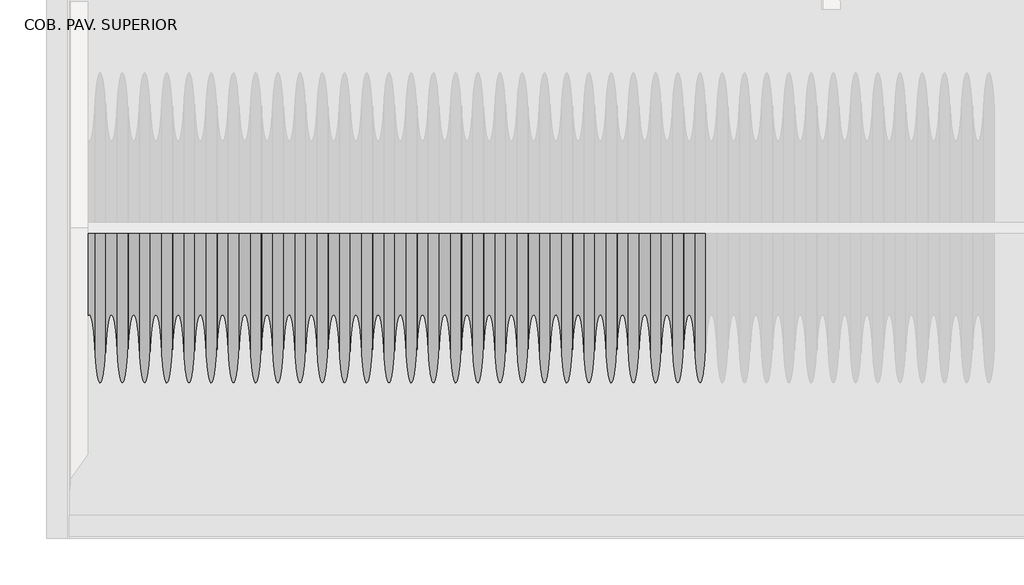
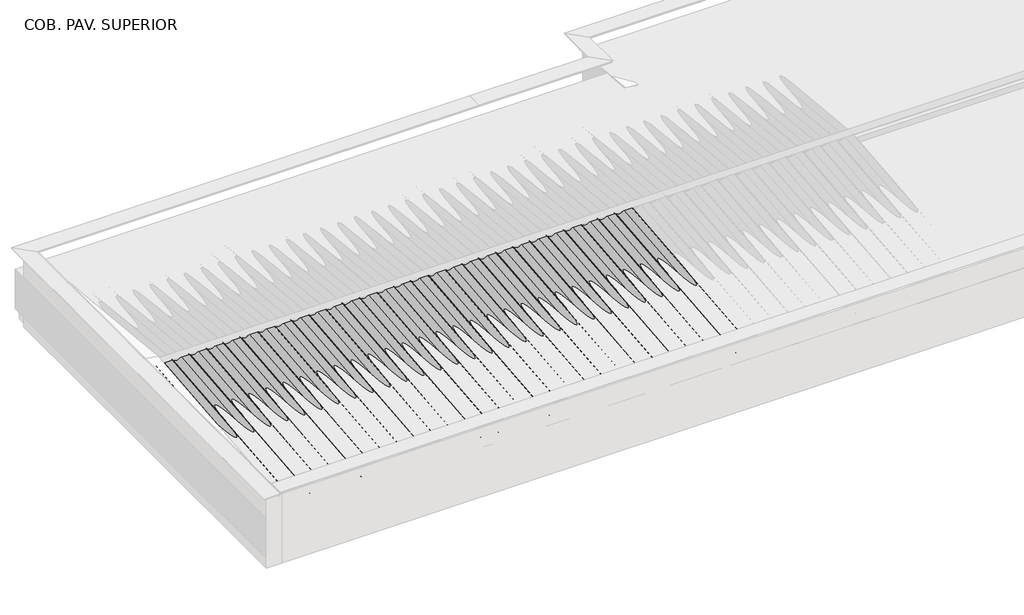
# One storey, part 2 of 8: 35 beams, 7 columns.
"""IFC4 building model written with IfcOpenShell, lengths in millimetres."""

import ifcopenshell
import ifcopenshell.guid

model = None  # the IFC model being written
_history = None  # IfcOwnerHistory: only IFC2X3 demands one
_inside = {}  # id of a spatial element -> (the spatial element, [elements in it])
_under = {}  # id of a project, library or spatial element -> (it, [spatial elements below it])
_declared = {}  # id of a project -> (the project, [libraries it declares])
_typed = {}  # id of a type object -> (the type object, [elements of that type])
_made_of = {}  # id of a material, layer set ... -> (it, [elements and type objects made of it])


def new_model(schema):
    """Start an empty IFC model of exactly this schema.

    Asked for "IFC4X3", IfcOpenShell would pick the latest addendum, in which some entities
    have other attributes; the version numbers below select the first issue.
    IFC2X3 requires an IfcOwnerHistory on every rooted entity: one is made here for all.
    """
    global model, _history
    if schema == "IFC4X3":
        model = ifcopenshell.file(schema_version=(4, 3, 0, 0))
    else:
        model = ifcopenshell.file(schema=schema)
    _inside.clear()
    _under.clear()
    _declared.clear()
    _typed.clear()
    _made_of.clear()
    _history = None
    if model.schema == "IFC2X3":
        org = make("IfcOrganization", Name="unknown")
        user = make(
            "IfcPersonAndOrganization",
            ThePerson=make("IfcPerson", FamilyName="unknown"),
            TheOrganization=org,
        )
        app = make(
            "IfcApplication",
            ApplicationDeveloper=org,
            Version="unknown",
            ApplicationFullName="unknown",
            ApplicationIdentifier="unknown",
        )
        _history = make(
            "IfcOwnerHistory",
            OwningUser=user,
            OwningApplication=app,
            ChangeAction="ADDED",
            CreationDate=0,
        )
    return model


def make(cls, **values):
    """One entity of the class cls with the attributes given. An attribute that is None is left unset."""
    return model.create_entity(
        cls, **{name: value for name, value in values.items() if value is not None}
    )


def rooted(cls, **values):
    """An entity with a GlobalId (a new one), such as an element, a storey or a relation."""
    return make(cls, GlobalId=ifcopenshell.guid.new(), OwnerHistory=_history, **values)


def si_unit(unit_type, name, prefix=None):
    """IfcSIUnit, for example si_unit("LENGTHUNIT", "METRE", prefix="MILLI")."""
    return make("IfcSIUnit", UnitType=unit_type, Prefix=prefix, Name=name)


def assignment(units):
    """IfcUnitAssignment: the units of a project."""
    return None if units is None else make("IfcUnitAssignment", Units=units)


def point(xyz):
    """IfcCartesianPoint."""
    return None if xyz is None else make("IfcCartesianPoint", Coordinates=xyz)


def direction(xyz):
    """IfcDirection."""
    return None if xyz is None else make("IfcDirection", DirectionRatios=xyz)


def frame(location, z_axis=None, x_axis=None):
    """IfcAxis2Placement3D, a coordinate frame: its origin and axes. An axis left out is left unset."""
    return make(
        "IfcAxis2Placement3D",
        Location=point(location),
        Axis=direction(z_axis),
        RefDirection=direction(x_axis),
    )


def frame_2d(location, x_axis=None):
    """IfcAxis2Placement2D, a coordinate frame in the plane: its origin and x axis."""
    return make(
        "IfcAxis2Placement2D", Location=point(location), RefDirection=direction(x_axis)
    )


def origin():
    """The frame at (0, 0, 0) with its axes left unset."""
    return frame((0.0, 0.0, 0.0))


def place(relative_to, where):
    """IfcLocalPlacement: puts the frame where relative to a parent placement (None: the world)."""
    return make(
        "IfcLocalPlacement", PlacementRelTo=relative_to, RelativePlacement=where
    )


def context(
    kind, dimensions, precision=None, world=None, true_north=None, identifier=None
):
    """IfcGeometricRepresentationContext, for example the 3D "Model" context."""
    return make(
        "IfcGeometricRepresentationContext",
        ContextIdentifier=identifier,
        ContextType=kind,
        CoordinateSpaceDimension=dimensions,
        Precision=precision,
        WorldCoordinateSystem=world,
        TrueNorth=true_north,
    )


def project(units=None, contexts=None):
    """IfcProject with its units and contexts."""
    return rooted(
        "IfcProject",
        Name="project",
        RepresentationContexts=contexts,
        UnitsInContext=assignment(units),
    )


def spatial(cls, under=None, at=None, **own):
    """A site, building, storey or space (cls), placed at a placement, below another one or the project."""
    s = rooted(cls, ObjectPlacement=at, **own)
    if under is not None:
        _under.setdefault(under.id(), (under, []))[1].append(s)
    return s


def polyline(points):
    """IfcPolyline through the points."""
    return make("IfcPolyline", Points=[point(p) for p in points])


def circle_curve(where, radius):
    """IfcCircle in the frame where."""
    return make("IfcCircle", Position=where, Radius=radius)


def trimmed(basis, trim1, trim2, sense, master):
    """IfcTrimmedCurve: the piece of a basis curve between two trims."""
    return make(
        "IfcTrimmedCurve",
        BasisCurve=basis,
        Trim1=trim1,
        Trim2=trim2,
        SenseAgreement=sense,
        MasterRepresentation=master,
    )


def segment(curve, same_sense, transition):
    """IfcCompositeCurveSegment."""
    return make(
        "IfcCompositeCurveSegment",
        Transition=transition,
        SameSense=same_sense,
        ParentCurve=curve,
    )


def composite_curve(segments, self_intersect=None):
    """IfcCompositeCurve: segments joined end to end."""
    return make("IfcCompositeCurve", Segments=segments, SelfIntersect=self_intersect)


def outline(outer, holes=None, kind="AREA"):
    """IfcArbitraryClosedProfileDef: a profile drawn as a closed curve; with holes, ...WithVoids."""
    if holes is None:
        return make("IfcArbitraryClosedProfileDef", ProfileType=kind, OuterCurve=outer)
    return make(
        "IfcArbitraryProfileDefWithVoids",
        ProfileType=kind,
        OuterCurve=outer,
        InnerCurves=holes,
    )


def extrude(swept, where, along, depth):
    """IfcExtrudedAreaSolid: the profile swept, set in the frame where, extruded along a direction by depth."""
    return make(
        "IfcExtrudedAreaSolid",
        SweptArea=swept,
        Position=where,
        ExtrudedDirection=direction(along),
        Depth=depth,
    )


def shape(context_of_items, identifier, shape_type, items):
    """IfcShapeRepresentation: the items that make up one representation, for example the "Body"."""
    return make(
        "IfcShapeRepresentation",
        ContextOfItems=context_of_items,
        RepresentationIdentifier=identifier,
        RepresentationType=shape_type,
        Items=items,
    )


def source(mapping_origin, context_of_items, identifier, shape_type, items):
    """IfcRepresentationMap: a shape defined once, which mapped items show again and again."""
    return make(
        "IfcRepresentationMap",
        MappingOrigin=mapping_origin,
        MappedRepresentation=shape(context_of_items, identifier, shape_type, items),
    )


def transform(
    local_origin,
    x_axis=None,
    y_axis=None,
    z_axis=None,
    scale=None,
    scale2=None,
    scale3=None,
    uniform=True,
):
    """IfcCartesianTransformationOperator3D, or its non-uniform kind. x_axis, y_axis, z_axis: its Axis1, 2, 3."""
    if uniform:
        return make(
            "IfcCartesianTransformationOperator3D",
            Axis1=direction(x_axis),
            Axis2=direction(y_axis),
            LocalOrigin=point(local_origin),
            Scale=scale,
            Axis3=direction(z_axis),
        )
    return make(
        "IfcCartesianTransformationOperator3DnonUniform",
        Axis1=direction(x_axis),
        Axis2=direction(y_axis),
        LocalOrigin=point(local_origin),
        Scale=scale,
        Axis3=direction(z_axis),
        Scale2=scale2,
        Scale3=scale3,
    )


def mapped(mapping_source, mapping_target):
    """IfcMappedItem: shows the shape of a source again, moved by a transform."""
    return make(
        "IfcMappedItem", MappingSource=mapping_source, MappingTarget=mapping_target
    )


def made_of(thing, what):
    """Note that an element or type object is made of a material, layer set ...; save() writes the relation."""
    if what is not None:
        _made_of.setdefault(what.id(), (what, []))[1].append(thing)
    return thing


def element(
    cls,
    number,
    at=None,
    inside=None,
    cuts=None,
    type_object=None,
    material=None,
    context=None,
    identifier="Body",
    shape_type=None,
    held_by="IfcProductDefinitionShape",
    body=None,
    shapes=None,
    **own,
):
    """One element of the class cls, such as IfcWall. Its Tag is "e" and its number.

    at: its placement. inside: the storey or other place that contains it. cuts: it is an
    opening in that element (IfcRelVoidsElement). A single representation is given by context,
    identifier, shape_type and body (its items); several are given by shapes. held_by: the class
    of the entity that holds the representations. save() writes the other relations.
    """
    e = rooted(cls, Tag="e%d" % number, ObjectPlacement=at, **own)
    if body is not None:
        shapes = [shape(context, identifier, shape_type, body)]
    if shapes is not None:
        e.Representation = make(held_by, Representations=shapes)
    if inside is not None:
        _inside.setdefault(inside.id(), (inside, []))[1].append(e)
    if cuts is not None:
        rooted(
            "IfcRelVoidsElement", RelatingBuildingElement=cuts, RelatedOpeningElement=e
        )
    if type_object is not None:
        _typed.setdefault(type_object.id(), (type_object, []))[1].append(e)
    return made_of(e, material)


def aggregate(whole, parts):
    """IfcRelAggregates: a whole, such as a stair, and the parts it consists of."""
    return rooted("IfcRelAggregates", RelatingObject=whole, RelatedObjects=parts)


def save(model, path):
    """Write the relations noted so far, then the file.

    IfcRelAggregates (storeys below a building ...), IfcRelContainedInSpatialStructure (elements
    in a storey), IfcRelDefinesByType, IfcRelAssociatesMaterial and IfcRelDeclares: one each for
    every whole, place, type object, material and project.
    """
    for whole, parts in _under.values():
        aggregate(whole, parts)
    for where, things in _inside.values():
        rooted(
            "IfcRelContainedInSpatialStructure",
            RelatedElements=things,
            RelatingStructure=where,
        )
    for kind, things in _typed.values():
        rooted("IfcRelDefinesByType", RelatedObjects=things, RelatingType=kind)
    for what, things in _made_of.values():
        rooted("IfcRelAssociatesMaterial", RelatedObjects=things, RelatingMaterial=what)
    for by, libraries in _declared.values():
        rooted("IfcRelDeclares", RelatingContext=by, RelatedDefinitions=libraries)
    model.write(path)


def beam_fe4ddbad(model_context):
    return source(origin(), model_context, "Body", "SweptSolid", [
        extrude(outline(polyline([(998.8971968, 30.0), (998.8971968, -30.0), (-998.8971974, -30.0), (-998.8971974, 30.0), (998.8971968, 30.0)])), frame((0.0, 0.0, -60.0), z_axis=(0.0, 0.0, 1.0), x_axis=(1.0, 0.0, 0.0)), (0.0, 0.0, 1.0), 120.0),
    ])


def column_6c15bf79(model_context):
    return source(origin(), model_context, "Body", "SweptSolid", [
        extrude(outline(polyline([(30.0, 80.0), (30.0, -80.0), (-30.0, -80.0), (-30.0, 80.0), (30.0, 80.0)])), frame((0.0, 0.0, 6710.0), z_axis=(0.0, 0.0, 1.0), x_axis=(1.0, 0.0, 0.0)), (0.0, 0.0, 1.0), 467.5),
    ])


def column_42eef9f8(model_context):
    return source(origin(), model_context, "Body", "SweptSolid", [
        extrude(outline(polyline([(30.0, 80.0), (30.0, -80.0), (-30.0, -80.0), (-30.0, 80.0), (30.0, 80.0)])), frame((0.0, 0.0, 6710.0), z_axis=(0.0, 0.0, 1.0), x_axis=(1.0, 0.0, 0.0)), (0.0, 0.0, 1.0), 227.1),
    ])


model = new_model("IFC4")

# Units and contexts
model_context = context("Model", 3, world=origin())
ifc_project = project(units=[si_unit("LENGTHUNIT", "METRE", prefix="MILLI")], contexts=[model_context])

# Site, building, storey
site = spatial("IfcSite", under=ifc_project)
building = spatial("IfcBuilding", under=site)
storey = spatial("IfcBuildingStorey", under=building, Name="COB. PAV. SUPERIOR", Elevation=6650.0)

# Beams
placement = place(None, origin())
beam_shape = beam_fe4ddbad(model_context)
element("IfcBeam", 1, ObjectType="Madeira de lei : Berço 6x12cm", at=placement, inside=storey, context=model_context, shape_type="MappedRepresentation", body=[
    mapped(beam_shape, transform((-11738.1841096, -9189.768869, 6680.0), x_axis=(1.0, 0.0, 0.0), y_axis=(0.0, 0.0, -1.0), z_axis=(0.0, 1.0, 0.0))),
])
element("IfcBeam", 2, ObjectType="Madeira de lei : Berço 6x12cm", at=placement, inside=storey, context=model_context, shape_type="MappedRepresentation", body=[
    mapped(beam_shape, transform((-11738.1841096, -10631.818869, 6680.0), x_axis=(1.0, 0.0, 0.0), y_axis=(0.0, 0.0, -1.0), z_axis=(0.0, 1.0, 0.0))),
])
element("IfcBeam", 3, ObjectType="Madeira de lei : Berço 6x12cm", at=placement, inside=storey, context=model_context, shape_type="MappedRepresentation", body=[
    mapped(beam_shape, transform((-9740.3897147, -9189.768869, 6680.0), x_axis=(1.0, 0.0, 0.0), y_axis=(0.0, 0.0, -1.0), z_axis=(0.0, 1.0, 0.0))),
])
element("IfcBeam", 4, ObjectType="Madeira de lei : Berço 6x12cm", at=placement, inside=storey, context=model_context, shape_type="MappedRepresentation", body=[
    mapped(beam_shape, transform((-7742.5953199, -9189.768869, 6680.0), x_axis=(1.0, 0.0, 0.0), y_axis=(0.0, 0.0, -1.0), z_axis=(0.0, 1.0, 0.0))),
])
element("IfcBeam", 5, ObjectType="Madeira de lei : Berço 6x12cm", at=placement, inside=storey, context=model_context, shape_type="MappedRepresentation", body=[
    mapped(beam_shape, transform((-9740.3897147, -10631.818869, 6680.0), x_axis=(1.0, 0.0, 0.0), y_axis=(0.0, 0.0, -1.0), z_axis=(0.0, 1.0, 0.0))),
])
element("IfcBeam", 6, ObjectType="Madeira de lei : Berço 6x12cm", at=placement, inside=storey, context=model_context, shape_type="MappedRepresentation", body=[
    mapped(beam_shape, transform((-7742.5953199, -10631.818869, 6680.0), x_axis=(1.0, 0.0, 0.0), y_axis=(0.0, 0.0, -1.0), z_axis=(0.0, 1.0, 0.0))),
])
element("IfcBeam", 7, ObjectType="Madeira de lei : Berço 6x12cm", at=placement, inside=storey, context=model_context, shape_type="MappedRepresentation", body=[
    mapped(beam_shape, transform((-5744.8009251, -10631.818869, 6680.0), x_axis=(1.0, 0.0, 0.0), y_axis=(0.0, 0.0, -1.0), z_axis=(0.0, 1.0, 0.0))),
])
element("IfcBeam", 8, ObjectType="Telha Ondulada : Fibrocimento", at=placement, inside=storey, context=model_context, shape_type="SweptSolid", body=[
    extrude(outline(composite_curve([segment(trimmed(circle_curve(frame_2d((0.0, 66.7939461)), 66.7939461), [point((29.3501489, 6.7939461))], [point((29.3501489, 126.7939461))], True, "CARTESIAN"), True, "CONTINUOUS"), segment(polyline([(29.3501489, 126.7939461), (31.5472154, 131.2853711)]), True, "CONTINUOUS"), segment(trimmed(circle_curve(frame_2d((0.0, 66.7939461)), 71.7939461), [point((31.5472154, 131.2853711))], [point((31.5472154, 2.3025211))], False, "CARTESIAN"), True, "CONTINUOUS"), segment(trimmed(circle_curve(frame_2d((58.7002978, -53.2060539)), 61.7939461), [point((31.5472154, 2.3025211))], [point((31.5472154, -108.7146289))], True, "CARTESIAN"), True, "CONTINUOUS"), segment(polyline([(31.5472154, -108.7146289), (29.3501489, -113.2060539)]), True, "CONTINUOUS"), segment(trimmed(circle_curve(frame_2d((58.7002978, -53.2060539)), 66.7939461), [point((29.3501489, -113.2060539))], [point((29.3501489, 6.7939461))], False, "CARTESIAN"), True, "CONTINUOUS")], self_intersect=False)), frame((-12452.7843743, -10831.9594023, 7106.8215886), z_axis=(0.0, 0.9950371902099894, 0.09950371902099749), x_axis=(0.0, 0.09950371902099749, -0.9950371902099894)), (0.0, 0.0, 1.0), 3060.4439799),
])
element("IfcBeam", 9, ObjectType="Telha Ondulada : Fibrocimento", at=placement, inside=storey, context=model_context, shape_type="SweptSolid", body=[
    extrude(outline(composite_curve([segment(trimmed(circle_curve(frame_2d((0.0, 66.7939461)), 66.7939461), [point((29.3501489, 6.7939461))], [point((29.3501489, 126.7939461))], True, "CARTESIAN"), True, "CONTINUOUS"), segment(polyline([(29.3501489, 126.7939461), (31.5472154, 131.2853711)]), True, "CONTINUOUS"), segment(trimmed(circle_curve(frame_2d((0.0, 66.7939461)), 71.7939461), [point((31.5472154, 131.2853711))], [point((31.5472154, 2.3025211))], False, "CARTESIAN"), True, "CONTINUOUS"), segment(trimmed(circle_curve(frame_2d((58.7002978, -53.2060539)), 61.7939461), [point((31.5472154, 2.3025211))], [point((31.5472154, -108.7146289))], True, "CARTESIAN"), True, "CONTINUOUS"), segment(polyline([(31.5472154, -108.7146289), (29.3501489, -113.2060539)]), True, "CONTINUOUS"), segment(trimmed(circle_curve(frame_2d((58.7002978, -53.2060539)), 66.7939461), [point((29.3501489, -113.2060539))], [point((29.3501489, 6.7939461))], False, "CARTESIAN"), True, "CONTINUOUS")], self_intersect=False)), frame((-12208.2843743, -10831.9594023, 7106.8215886), z_axis=(0.0, 0.9950371902099894, 0.09950371902099749), x_axis=(0.0, 0.09950371902099749, -0.9950371902099894)), (0.0, 0.0, 1.0), 3060.4439799),
])
element("IfcBeam", 10, ObjectType="Telha Ondulada : Fibrocimento", at=placement, inside=storey, context=model_context, shape_type="SweptSolid", body=[
    extrude(outline(composite_curve([segment(trimmed(circle_curve(frame_2d((0.0, 66.7939461)), 66.7939461), [point((29.3501489, 6.7939461))], [point((29.3501489, 126.7939461))], True, "CARTESIAN"), True, "CONTINUOUS"), segment(polyline([(29.3501489, 126.7939461), (31.5472154, 131.2853711)]), True, "CONTINUOUS"), segment(trimmed(circle_curve(frame_2d((0.0, 66.7939461)), 71.7939461), [point((31.5472154, 131.2853711))], [point((31.5472154, 2.3025211))], False, "CARTESIAN"), True, "CONTINUOUS"), segment(trimmed(circle_curve(frame_2d((58.7002978, -53.2060539)), 61.7939461), [point((31.5472154, 2.3025211))], [point((31.5472154, -108.7146289))], True, "CARTESIAN"), True, "CONTINUOUS"), segment(polyline([(31.5472154, -108.7146289), (29.3501489, -113.2060539)]), True, "CONTINUOUS"), segment(trimmed(circle_curve(frame_2d((58.7002978, -53.2060539)), 66.7939461), [point((29.3501489, -113.2060539))], [point((29.3501489, 6.7939461))], False, "CARTESIAN"), True, "CONTINUOUS")], self_intersect=False)), frame((-11963.7843743, -10831.9594023, 7106.8215886), z_axis=(0.0, 0.9950371902099894, 0.09950371902099749), x_axis=(0.0, 0.09950371902099749, -0.9950371902099894)), (0.0, 0.0, 1.0), 3060.4439799),
])
element("IfcBeam", 11, ObjectType="Telha Ondulada : Fibrocimento", at=placement, inside=storey, context=model_context, shape_type="SweptSolid", body=[
    extrude(outline(composite_curve([segment(trimmed(circle_curve(frame_2d((0.0, 66.7939461)), 66.7939461), [point((29.3501489, 6.7939461))], [point((29.3501489, 126.7939461))], True, "CARTESIAN"), True, "CONTINUOUS"), segment(polyline([(29.3501489, 126.7939461), (31.5472154, 131.2853711)]), True, "CONTINUOUS"), segment(trimmed(circle_curve(frame_2d((0.0, 66.7939461)), 71.7939461), [point((31.5472154, 131.2853711))], [point((31.5472154, 2.3025211))], False, "CARTESIAN"), True, "CONTINUOUS"), segment(trimmed(circle_curve(frame_2d((58.7002978, -53.2060539)), 61.7939461), [point((31.5472154, 2.3025211))], [point((31.5472154, -108.7146289))], True, "CARTESIAN"), True, "CONTINUOUS"), segment(polyline([(31.5472154, -108.7146289), (29.3501489, -113.2060539)]), True, "CONTINUOUS"), segment(trimmed(circle_curve(frame_2d((58.7002978, -53.2060539)), 66.7939461), [point((29.3501489, -113.2060539))], [point((29.3501489, 6.7939461))], False, "CARTESIAN"), True, "CONTINUOUS")], self_intersect=False)), frame((-11719.2843743, -10831.9594023, 7106.8215886), z_axis=(0.0, 0.9950371902099894, 0.09950371902099749), x_axis=(0.0, 0.09950371902099749, -0.9950371902099894)), (0.0, 0.0, 1.0), 3060.4439799),
])
element("IfcBeam", 12, ObjectType="Telha Ondulada : Fibrocimento", at=placement, inside=storey, context=model_context, shape_type="SweptSolid", body=[
    extrude(outline(composite_curve([segment(trimmed(circle_curve(frame_2d((0.0, 66.7939461)), 66.7939461), [point((29.3501489, 6.7939461))], [point((29.3501489, 126.7939461))], True, "CARTESIAN"), True, "CONTINUOUS"), segment(polyline([(29.3501489, 126.7939461), (31.5472154, 131.2853711)]), True, "CONTINUOUS"), segment(trimmed(circle_curve(frame_2d((0.0, 66.7939461)), 71.7939461), [point((31.5472154, 131.2853711))], [point((31.5472154, 2.3025211))], False, "CARTESIAN"), True, "CONTINUOUS"), segment(trimmed(circle_curve(frame_2d((58.7002978, -53.2060539)), 61.7939461), [point((31.5472154, 2.3025211))], [point((31.5472154, -108.7146289))], True, "CARTESIAN"), True, "CONTINUOUS"), segment(polyline([(31.5472154, -108.7146289), (29.3501489, -113.2060539)]), True, "CONTINUOUS"), segment(trimmed(circle_curve(frame_2d((58.7002978, -53.2060539)), 66.7939461), [point((29.3501489, -113.2060539))], [point((29.3501489, 6.7939461))], False, "CARTESIAN"), True, "CONTINUOUS")], self_intersect=False)), frame((-11474.7843743, -10831.9594023, 7106.8215886), z_axis=(0.0, 0.9950371902099894, 0.09950371902099749), x_axis=(0.0, 0.09950371902099749, -0.9950371902099894)), (0.0, 0.0, 1.0), 3060.4439799),
])
element("IfcBeam", 13, ObjectType="Telha Ondulada : Fibrocimento", at=placement, inside=storey, context=model_context, shape_type="SweptSolid", body=[
    extrude(outline(composite_curve([segment(trimmed(circle_curve(frame_2d((0.0, 66.7939461)), 66.7939461), [point((29.3501489, 6.7939461))], [point((29.3501489, 126.7939461))], True, "CARTESIAN"), True, "CONTINUOUS"), segment(polyline([(29.3501489, 126.7939461), (31.5472154, 131.2853711)]), True, "CONTINUOUS"), segment(trimmed(circle_curve(frame_2d((0.0, 66.7939461)), 71.7939461), [point((31.5472154, 131.2853711))], [point((31.5472154, 2.3025211))], False, "CARTESIAN"), True, "CONTINUOUS"), segment(trimmed(circle_curve(frame_2d((58.7002978, -53.2060539)), 61.7939461), [point((31.5472154, 2.3025211))], [point((31.5472154, -108.7146289))], True, "CARTESIAN"), True, "CONTINUOUS"), segment(polyline([(31.5472154, -108.7146289), (29.3501489, -113.2060539)]), True, "CONTINUOUS"), segment(trimmed(circle_curve(frame_2d((58.7002978, -53.2060539)), 66.7939461), [point((29.3501489, -113.2060539))], [point((29.3501489, 6.7939461))], False, "CARTESIAN"), True, "CONTINUOUS")], self_intersect=False)), frame((-11230.2843743, -10831.9594023, 7106.8215886), z_axis=(0.0, 0.9950371902099894, 0.09950371902099749), x_axis=(0.0, 0.09950371902099749, -0.9950371902099894)), (0.0, 0.0, 1.0), 3060.4439799),
])
element("IfcBeam", 14, ObjectType="Telha Ondulada : Fibrocimento", at=placement, inside=storey, context=model_context, shape_type="SweptSolid", body=[
    extrude(outline(composite_curve([segment(trimmed(circle_curve(frame_2d((0.0, 66.7939461)), 66.7939461), [point((29.3501489, 6.7939461))], [point((29.3501489, 126.7939461))], True, "CARTESIAN"), True, "CONTINUOUS"), segment(polyline([(29.3501489, 126.7939461), (31.5472154, 131.2853711)]), True, "CONTINUOUS"), segment(trimmed(circle_curve(frame_2d((0.0, 66.7939461)), 71.7939461), [point((31.5472154, 131.2853711))], [point((31.5472154, 2.3025211))], False, "CARTESIAN"), True, "CONTINUOUS"), segment(trimmed(circle_curve(frame_2d((58.7002978, -53.2060539)), 61.7939461), [point((31.5472154, 2.3025211))], [point((31.5472154, -108.7146289))], True, "CARTESIAN"), True, "CONTINUOUS"), segment(polyline([(31.5472154, -108.7146289), (29.3501489, -113.2060539)]), True, "CONTINUOUS"), segment(trimmed(circle_curve(frame_2d((58.7002978, -53.2060539)), 66.7939461), [point((29.3501489, -113.2060539))], [point((29.3501489, 6.7939461))], False, "CARTESIAN"), True, "CONTINUOUS")], self_intersect=False)), frame((-10985.7843743, -10831.9594023, 7106.8215886), z_axis=(0.0, 0.9950371902099894, 0.09950371902099749), x_axis=(0.0, 0.09950371902099749, -0.9950371902099894)), (0.0, 0.0, 1.0), 3060.4439799),
])
element("IfcBeam", 15, ObjectType="Telha Ondulada : Fibrocimento", at=placement, inside=storey, context=model_context, shape_type="SweptSolid", body=[
    extrude(outline(composite_curve([segment(trimmed(circle_curve(frame_2d((0.0, 66.7939461)), 66.7939461), [point((29.3501489, 6.7939461))], [point((29.3501489, 126.7939461))], True, "CARTESIAN"), True, "CONTINUOUS"), segment(polyline([(29.3501489, 126.7939461), (31.5472154, 131.2853711)]), True, "CONTINUOUS"), segment(trimmed(circle_curve(frame_2d((0.0, 66.7939461)), 71.7939461), [point((31.5472154, 131.2853711))], [point((31.5472154, 2.3025211))], False, "CARTESIAN"), True, "CONTINUOUS"), segment(trimmed(circle_curve(frame_2d((58.7002978, -53.2060539)), 61.7939461), [point((31.5472154, 2.3025211))], [point((31.5472154, -108.7146289))], True, "CARTESIAN"), True, "CONTINUOUS"), segment(polyline([(31.5472154, -108.7146289), (29.3501489, -113.2060539)]), True, "CONTINUOUS"), segment(trimmed(circle_curve(frame_2d((58.7002978, -53.2060539)), 66.7939461), [point((29.3501489, -113.2060539))], [point((29.3501489, 6.7939461))], False, "CARTESIAN"), True, "CONTINUOUS")], self_intersect=False)), frame((-10741.2843743, -10831.9594023, 7106.8215886), z_axis=(0.0, 0.9950371902099894, 0.09950371902099749), x_axis=(0.0, 0.09950371902099749, -0.9950371902099894)), (0.0, 0.0, 1.0), 3060.4439799),
])
element("IfcBeam", 16, ObjectType="Telha Ondulada : Fibrocimento", at=placement, inside=storey, context=model_context, shape_type="SweptSolid", body=[
    extrude(outline(composite_curve([segment(trimmed(circle_curve(frame_2d((0.0, 66.7939461)), 66.7939461), [point((29.3501489, 6.7939461))], [point((29.3501489, 126.7939461))], True, "CARTESIAN"), True, "CONTINUOUS"), segment(polyline([(29.3501489, 126.7939461), (31.5472154, 131.2853711)]), True, "CONTINUOUS"), segment(trimmed(circle_curve(frame_2d((0.0, 66.7939461)), 71.7939461), [point((31.5472154, 131.2853711))], [point((31.5472154, 2.3025211))], False, "CARTESIAN"), True, "CONTINUOUS"), segment(trimmed(circle_curve(frame_2d((58.7002978, -53.2060539)), 61.7939461), [point((31.5472154, 2.3025211))], [point((31.5472154, -108.7146289))], True, "CARTESIAN"), True, "CONTINUOUS"), segment(polyline([(31.5472154, -108.7146289), (29.3501489, -113.2060539)]), True, "CONTINUOUS"), segment(trimmed(circle_curve(frame_2d((58.7002978, -53.2060539)), 66.7939461), [point((29.3501489, -113.2060539))], [point((29.3501489, 6.7939461))], False, "CARTESIAN"), True, "CONTINUOUS")], self_intersect=False)), frame((-10496.7843743, -10831.9594023, 7106.8215886), z_axis=(0.0, 0.9950371902099894, 0.09950371902099749), x_axis=(0.0, 0.09950371902099749, -0.9950371902099894)), (0.0, 0.0, 1.0), 3060.4439799),
])
element("IfcBeam", 17, ObjectType="Telha Ondulada : Fibrocimento", at=placement, inside=storey, context=model_context, shape_type="SweptSolid", body=[
    extrude(outline(composite_curve([segment(trimmed(circle_curve(frame_2d((0.0, 66.7939461)), 66.7939461), [point((29.3501489, 6.7939461))], [point((29.3501489, 126.7939461))], True, "CARTESIAN"), True, "CONTINUOUS"), segment(polyline([(29.3501489, 126.7939461), (31.5472154, 131.2853711)]), True, "CONTINUOUS"), segment(trimmed(circle_curve(frame_2d((0.0, 66.7939461)), 71.7939461), [point((31.5472154, 131.2853711))], [point((31.5472154, 2.3025211))], False, "CARTESIAN"), True, "CONTINUOUS"), segment(trimmed(circle_curve(frame_2d((58.7002978, -53.2060539)), 61.7939461), [point((31.5472154, 2.3025211))], [point((31.5472154, -108.7146289))], True, "CARTESIAN"), True, "CONTINUOUS"), segment(polyline([(31.5472154, -108.7146289), (29.3501489, -113.2060539)]), True, "CONTINUOUS"), segment(trimmed(circle_curve(frame_2d((58.7002978, -53.2060539)), 66.7939461), [point((29.3501489, -113.2060539))], [point((29.3501489, 6.7939461))], False, "CARTESIAN"), True, "CONTINUOUS")], self_intersect=False)), frame((-10252.2843743, -10831.9594023, 7106.8215886), z_axis=(0.0, 0.9950371902099894, 0.09950371902099749), x_axis=(0.0, 0.09950371902099749, -0.9950371902099894)), (0.0, 0.0, 1.0), 3060.4439799),
])
element("IfcBeam", 18, ObjectType="Telha Ondulada : Fibrocimento", at=placement, inside=storey, context=model_context, shape_type="SweptSolid", body=[
    extrude(outline(composite_curve([segment(trimmed(circle_curve(frame_2d((0.0, 66.7939461)), 66.7939461), [point((29.3501489, 6.7939461))], [point((29.3501489, 126.7939461))], True, "CARTESIAN"), True, "CONTINUOUS"), segment(polyline([(29.3501489, 126.7939461), (31.5472154, 131.2853711)]), True, "CONTINUOUS"), segment(trimmed(circle_curve(frame_2d((0.0, 66.7939461)), 71.7939461), [point((31.5472154, 131.2853711))], [point((31.5472154, 2.3025211))], False, "CARTESIAN"), True, "CONTINUOUS"), segment(trimmed(circle_curve(frame_2d((58.7002978, -53.2060539)), 61.7939461), [point((31.5472154, 2.3025211))], [point((31.5472154, -108.7146289))], True, "CARTESIAN"), True, "CONTINUOUS"), segment(polyline([(31.5472154, -108.7146289), (29.3501489, -113.2060539)]), True, "CONTINUOUS"), segment(trimmed(circle_curve(frame_2d((58.7002978, -53.2060539)), 66.7939461), [point((29.3501489, -113.2060539))], [point((29.3501489, 6.7939461))], False, "CARTESIAN"), True, "CONTINUOUS")], self_intersect=False)), frame((-10007.7843743, -10831.9594023, 7106.8215886), z_axis=(0.0, 0.9950371902099894, 0.09950371902099749), x_axis=(0.0, 0.09950371902099749, -0.9950371902099894)), (0.0, 0.0, 1.0), 3060.4439799),
])
element("IfcBeam", 19, ObjectType="Telha Ondulada : Fibrocimento", at=placement, inside=storey, context=model_context, shape_type="SweptSolid", body=[
    extrude(outline(composite_curve([segment(trimmed(circle_curve(frame_2d((0.0, 66.7939461)), 66.7939461), [point((29.3501489, 6.7939461))], [point((29.3501489, 126.7939461))], True, "CARTESIAN"), True, "CONTINUOUS"), segment(polyline([(29.3501489, 126.7939461), (31.5472154, 131.2853711)]), True, "CONTINUOUS"), segment(trimmed(circle_curve(frame_2d((0.0, 66.7939461)), 71.7939461), [point((31.5472154, 131.2853711))], [point((31.5472154, 2.3025211))], False, "CARTESIAN"), True, "CONTINUOUS"), segment(trimmed(circle_curve(frame_2d((58.7002978, -53.2060539)), 61.7939461), [point((31.5472154, 2.3025211))], [point((31.5472154, -108.7146289))], True, "CARTESIAN"), True, "CONTINUOUS"), segment(polyline([(31.5472154, -108.7146289), (29.3501489, -113.2060539)]), True, "CONTINUOUS"), segment(trimmed(circle_curve(frame_2d((58.7002978, -53.2060539)), 66.7939461), [point((29.3501489, -113.2060539))], [point((29.3501489, 6.7939461))], False, "CARTESIAN"), True, "CONTINUOUS")], self_intersect=False)), frame((-9763.2843743, -10831.9594023, 7106.8215886), z_axis=(0.0, 0.9950371902099894, 0.09950371902099749), x_axis=(0.0, 0.09950371902099749, -0.9950371902099894)), (0.0, 0.0, 1.0), 3060.4439799),
])
element("IfcBeam", 20, ObjectType="Telha Ondulada : Fibrocimento", at=placement, inside=storey, context=model_context, shape_type="SweptSolid", body=[
    extrude(outline(composite_curve([segment(trimmed(circle_curve(frame_2d((0.0, 66.7939461)), 66.7939461), [point((29.3501489, 6.7939461))], [point((29.3501489, 126.7939461))], True, "CARTESIAN"), True, "CONTINUOUS"), segment(polyline([(29.3501489, 126.7939461), (31.5472154, 131.2853711)]), True, "CONTINUOUS"), segment(trimmed(circle_curve(frame_2d((0.0, 66.7939461)), 71.7939461), [point((31.5472154, 131.2853711))], [point((31.5472154, 2.3025211))], False, "CARTESIAN"), True, "CONTINUOUS"), segment(trimmed(circle_curve(frame_2d((58.7002978, -53.2060539)), 61.7939461), [point((31.5472154, 2.3025211))], [point((31.5472154, -108.7146289))], True, "CARTESIAN"), True, "CONTINUOUS"), segment(polyline([(31.5472154, -108.7146289), (29.3501489, -113.2060539)]), True, "CONTINUOUS"), segment(trimmed(circle_curve(frame_2d((58.7002978, -53.2060539)), 66.7939461), [point((29.3501489, -113.2060539))], [point((29.3501489, 6.7939461))], False, "CARTESIAN"), True, "CONTINUOUS")], self_intersect=False)), frame((-9518.7843743, -10831.9594023, 7106.8215886), z_axis=(0.0, 0.9950371902099894, 0.09950371902099749), x_axis=(0.0, 0.09950371902099749, -0.9950371902099894)), (0.0, 0.0, 1.0), 3060.4439799),
])
element("IfcBeam", 21, ObjectType="Telha Ondulada : Fibrocimento", at=placement, inside=storey, context=model_context, shape_type="SweptSolid", body=[
    extrude(outline(composite_curve([segment(trimmed(circle_curve(frame_2d((0.0, 66.7939461)), 66.7939461), [point((29.3501489, 6.7939461))], [point((29.3501489, 126.7939461))], True, "CARTESIAN"), True, "CONTINUOUS"), segment(polyline([(29.3501489, 126.7939461), (31.5472154, 131.2853711)]), True, "CONTINUOUS"), segment(trimmed(circle_curve(frame_2d((0.0, 66.7939461)), 71.7939461), [point((31.5472154, 131.2853711))], [point((31.5472154, 2.3025211))], False, "CARTESIAN"), True, "CONTINUOUS"), segment(trimmed(circle_curve(frame_2d((58.7002978, -53.2060539)), 61.7939461), [point((31.5472154, 2.3025211))], [point((31.5472154, -108.7146289))], True, "CARTESIAN"), True, "CONTINUOUS"), segment(polyline([(31.5472154, -108.7146289), (29.3501489, -113.2060539)]), True, "CONTINUOUS"), segment(trimmed(circle_curve(frame_2d((58.7002978, -53.2060539)), 66.7939461), [point((29.3501489, -113.2060539))], [point((29.3501489, 6.7939461))], False, "CARTESIAN"), True, "CONTINUOUS")], self_intersect=False)), frame((-9274.2843743, -10831.9594023, 7106.8215886), z_axis=(0.0, 0.9950371902099894, 0.09950371902099749), x_axis=(0.0, 0.09950371902099749, -0.9950371902099894)), (0.0, 0.0, 1.0), 3060.4439799),
])
element("IfcBeam", 22, ObjectType="Telha Ondulada : Fibrocimento", at=placement, inside=storey, context=model_context, shape_type="SweptSolid", body=[
    extrude(outline(composite_curve([segment(trimmed(circle_curve(frame_2d((0.0, 66.7939461)), 66.7939461), [point((29.3501489, 6.7939461))], [point((29.3501489, 126.7939461))], True, "CARTESIAN"), True, "CONTINUOUS"), segment(polyline([(29.3501489, 126.7939461), (31.5472154, 131.2853711)]), True, "CONTINUOUS"), segment(trimmed(circle_curve(frame_2d((0.0, 66.7939461)), 71.7939461), [point((31.5472154, 131.2853711))], [point((31.5472154, 2.3025211))], False, "CARTESIAN"), True, "CONTINUOUS"), segment(trimmed(circle_curve(frame_2d((58.7002978, -53.2060539)), 61.7939461), [point((31.5472154, 2.3025211))], [point((31.5472154, -108.7146289))], True, "CARTESIAN"), True, "CONTINUOUS"), segment(polyline([(31.5472154, -108.7146289), (29.3501489, -113.2060539)]), True, "CONTINUOUS"), segment(trimmed(circle_curve(frame_2d((58.7002978, -53.2060539)), 66.7939461), [point((29.3501489, -113.2060539))], [point((29.3501489, 6.7939461))], False, "CARTESIAN"), True, "CONTINUOUS")], self_intersect=False)), frame((-9029.7843743, -10831.9594023, 7106.8215886), z_axis=(0.0, 0.9950371902099894, 0.09950371902099749), x_axis=(0.0, 0.09950371902099749, -0.9950371902099894)), (0.0, 0.0, 1.0), 3060.4439799),
])
element("IfcBeam", 23, ObjectType="Telha Ondulada : Fibrocimento", at=placement, inside=storey, context=model_context, shape_type="SweptSolid", body=[
    extrude(outline(composite_curve([segment(trimmed(circle_curve(frame_2d((0.0, 66.7939461)), 66.7939461), [point((29.3501489, 6.7939461))], [point((29.3501489, 126.7939461))], True, "CARTESIAN"), True, "CONTINUOUS"), segment(polyline([(29.3501489, 126.7939461), (31.5472154, 131.2853711)]), True, "CONTINUOUS"), segment(trimmed(circle_curve(frame_2d((0.0, 66.7939461)), 71.7939461), [point((31.5472154, 131.2853711))], [point((31.5472154, 2.3025211))], False, "CARTESIAN"), True, "CONTINUOUS"), segment(trimmed(circle_curve(frame_2d((58.7002978, -53.2060539)), 61.7939461), [point((31.5472154, 2.3025211))], [point((31.5472154, -108.7146289))], True, "CARTESIAN"), True, "CONTINUOUS"), segment(polyline([(31.5472154, -108.7146289), (29.3501489, -113.2060539)]), True, "CONTINUOUS"), segment(trimmed(circle_curve(frame_2d((58.7002978, -53.2060539)), 66.7939461), [point((29.3501489, -113.2060539))], [point((29.3501489, 6.7939461))], False, "CARTESIAN"), True, "CONTINUOUS")], self_intersect=False)), frame((-8785.2843743, -10831.9594023, 7106.8215886), z_axis=(0.0, 0.9950371902099894, 0.09950371902099749), x_axis=(0.0, 0.09950371902099749, -0.9950371902099894)), (0.0, 0.0, 1.0), 3060.4439799),
])
element("IfcBeam", 24, ObjectType="Telha Ondulada : Fibrocimento", at=placement, inside=storey, context=model_context, shape_type="SweptSolid", body=[
    extrude(outline(composite_curve([segment(trimmed(circle_curve(frame_2d((0.0, 66.7939461)), 66.7939461), [point((29.3501489, 6.7939461))], [point((29.3501489, 126.7939461))], True, "CARTESIAN"), True, "CONTINUOUS"), segment(polyline([(29.3501489, 126.7939461), (31.5472154, 131.2853711)]), True, "CONTINUOUS"), segment(trimmed(circle_curve(frame_2d((0.0, 66.7939461)), 71.7939461), [point((31.5472154, 131.2853711))], [point((31.5472154, 2.3025211))], False, "CARTESIAN"), True, "CONTINUOUS"), segment(trimmed(circle_curve(frame_2d((58.7002978, -53.2060539)), 61.7939461), [point((31.5472154, 2.3025211))], [point((31.5472154, -108.7146289))], True, "CARTESIAN"), True, "CONTINUOUS"), segment(polyline([(31.5472154, -108.7146289), (29.3501489, -113.2060539)]), True, "CONTINUOUS"), segment(trimmed(circle_curve(frame_2d((58.7002978, -53.2060539)), 66.7939461), [point((29.3501489, -113.2060539))], [point((29.3501489, 6.7939461))], False, "CARTESIAN"), True, "CONTINUOUS")], self_intersect=False)), frame((-8540.7843743, -10831.9594023, 7106.8215886), z_axis=(0.0, 0.9950371902099894, 0.09950371902099749), x_axis=(0.0, 0.09950371902099749, -0.9950371902099894)), (0.0, 0.0, 1.0), 3060.4439799),
])
element("IfcBeam", 25, ObjectType="Telha Ondulada : Fibrocimento", at=placement, inside=storey, context=model_context, shape_type="SweptSolid", body=[
    extrude(outline(composite_curve([segment(trimmed(circle_curve(frame_2d((0.0, 66.7939461)), 66.7939461), [point((29.3501489, 6.7939461))], [point((29.3501489, 126.7939461))], True, "CARTESIAN"), True, "CONTINUOUS"), segment(polyline([(29.3501489, 126.7939461), (31.5472154, 131.2853711)]), True, "CONTINUOUS"), segment(trimmed(circle_curve(frame_2d((0.0, 66.7939461)), 71.7939461), [point((31.5472154, 131.2853711))], [point((31.5472154, 2.3025211))], False, "CARTESIAN"), True, "CONTINUOUS"), segment(trimmed(circle_curve(frame_2d((58.7002978, -53.2060539)), 61.7939461), [point((31.5472154, 2.3025211))], [point((31.5472154, -108.7146289))], True, "CARTESIAN"), True, "CONTINUOUS"), segment(polyline([(31.5472154, -108.7146289), (29.3501489, -113.2060539)]), True, "CONTINUOUS"), segment(trimmed(circle_curve(frame_2d((58.7002978, -53.2060539)), 66.7939461), [point((29.3501489, -113.2060539))], [point((29.3501489, 6.7939461))], False, "CARTESIAN"), True, "CONTINUOUS")], self_intersect=False)), frame((-8296.2843743, -10831.9594023, 7106.8215886), z_axis=(0.0, 0.9950371902099894, 0.09950371902099749), x_axis=(0.0, 0.09950371902099749, -0.9950371902099894)), (0.0, 0.0, 1.0), 3060.4439799),
])
element("IfcBeam", 26, ObjectType="Telha Ondulada : Fibrocimento", at=placement, inside=storey, context=model_context, shape_type="SweptSolid", body=[
    extrude(outline(composite_curve([segment(trimmed(circle_curve(frame_2d((0.0, 66.7939461)), 66.7939461), [point((29.3501489, 6.7939461))], [point((29.3501489, 126.7939461))], True, "CARTESIAN"), True, "CONTINUOUS"), segment(polyline([(29.3501489, 126.7939461), (31.5472154, 131.2853711)]), True, "CONTINUOUS"), segment(trimmed(circle_curve(frame_2d((0.0, 66.7939461)), 71.7939461), [point((31.5472154, 131.2853711))], [point((31.5472154, 2.3025211))], False, "CARTESIAN"), True, "CONTINUOUS"), segment(trimmed(circle_curve(frame_2d((58.7002978, -53.2060539)), 61.7939461), [point((31.5472154, 2.3025211))], [point((31.5472154, -108.7146289))], True, "CARTESIAN"), True, "CONTINUOUS"), segment(polyline([(31.5472154, -108.7146289), (29.3501489, -113.2060539)]), True, "CONTINUOUS"), segment(trimmed(circle_curve(frame_2d((58.7002978, -53.2060539)), 66.7939461), [point((29.3501489, -113.2060539))], [point((29.3501489, 6.7939461))], False, "CARTESIAN"), True, "CONTINUOUS")], self_intersect=False)), frame((-8051.7843743, -10831.9594023, 7106.8215886), z_axis=(0.0, 0.9950371902099894, 0.09950371902099749), x_axis=(0.0, 0.09950371902099749, -0.9950371902099894)), (0.0, 0.0, 1.0), 3060.4439799),
])
element("IfcBeam", 27, ObjectType="Telha Ondulada : Fibrocimento", at=placement, inside=storey, context=model_context, shape_type="SweptSolid", body=[
    extrude(outline(composite_curve([segment(trimmed(circle_curve(frame_2d((0.0, 66.7939461)), 66.7939461), [point((29.3501489, 6.7939461))], [point((29.3501489, 126.7939461))], True, "CARTESIAN"), True, "CONTINUOUS"), segment(polyline([(29.3501489, 126.7939461), (31.5472154, 131.2853711)]), True, "CONTINUOUS"), segment(trimmed(circle_curve(frame_2d((0.0, 66.7939461)), 71.7939461), [point((31.5472154, 131.2853711))], [point((31.5472154, 2.3025211))], False, "CARTESIAN"), True, "CONTINUOUS"), segment(trimmed(circle_curve(frame_2d((58.7002978, -53.2060539)), 61.7939461), [point((31.5472154, 2.3025211))], [point((31.5472154, -108.7146289))], True, "CARTESIAN"), True, "CONTINUOUS"), segment(polyline([(31.5472154, -108.7146289), (29.3501489, -113.2060539)]), True, "CONTINUOUS"), segment(trimmed(circle_curve(frame_2d((58.7002978, -53.2060539)), 66.7939461), [point((29.3501489, -113.2060539))], [point((29.3501489, 6.7939461))], False, "CARTESIAN"), True, "CONTINUOUS")], self_intersect=False)), frame((-7807.2843743, -10831.9594023, 7106.8215886), z_axis=(0.0, 0.9950371902099894, 0.09950371902099749), x_axis=(0.0, 0.09950371902099749, -0.9950371902099894)), (0.0, 0.0, 1.0), 3060.4439799),
])
element("IfcBeam", 28, ObjectType="Telha Ondulada : Fibrocimento", at=placement, inside=storey, context=model_context, shape_type="SweptSolid", body=[
    extrude(outline(composite_curve([segment(trimmed(circle_curve(frame_2d((0.0, 66.7939461)), 66.7939461), [point((29.3501489, 6.7939461))], [point((29.3501489, 126.7939461))], True, "CARTESIAN"), True, "CONTINUOUS"), segment(polyline([(29.3501489, 126.7939461), (31.5472154, 131.2853711)]), True, "CONTINUOUS"), segment(trimmed(circle_curve(frame_2d((0.0, 66.7939461)), 71.7939461), [point((31.5472154, 131.2853711))], [point((31.5472154, 2.3025211))], False, "CARTESIAN"), True, "CONTINUOUS"), segment(trimmed(circle_curve(frame_2d((58.7002978, -53.2060539)), 61.7939461), [point((31.5472154, 2.3025211))], [point((31.5472154, -108.7146289))], True, "CARTESIAN"), True, "CONTINUOUS"), segment(polyline([(31.5472154, -108.7146289), (29.3501489, -113.2060539)]), True, "CONTINUOUS"), segment(trimmed(circle_curve(frame_2d((58.7002978, -53.2060539)), 66.7939461), [point((29.3501489, -113.2060539))], [point((29.3501489, 6.7939461))], False, "CARTESIAN"), True, "CONTINUOUS")], self_intersect=False)), frame((-7562.7843743, -10831.9594023, 7106.8215886), z_axis=(0.0, 0.9950371902099894, 0.09950371902099749), x_axis=(0.0, 0.09950371902099749, -0.9950371902099894)), (0.0, 0.0, 1.0), 3060.4439799),
])
element("IfcBeam", 29, ObjectType="Telha Ondulada : Fibrocimento", at=placement, inside=storey, context=model_context, shape_type="SweptSolid", body=[
    extrude(outline(composite_curve([segment(trimmed(circle_curve(frame_2d((0.0, 66.7939461)), 66.7939461), [point((29.3501489, 6.7939461))], [point((29.3501489, 126.7939461))], True, "CARTESIAN"), True, "CONTINUOUS"), segment(polyline([(29.3501489, 126.7939461), (31.5472154, 131.2853711)]), True, "CONTINUOUS"), segment(trimmed(circle_curve(frame_2d((0.0, 66.7939461)), 71.7939461), [point((31.5472154, 131.2853711))], [point((31.5472154, 2.3025211))], False, "CARTESIAN"), True, "CONTINUOUS"), segment(trimmed(circle_curve(frame_2d((58.7002978, -53.2060539)), 61.7939461), [point((31.5472154, 2.3025211))], [point((31.5472154, -108.7146289))], True, "CARTESIAN"), True, "CONTINUOUS"), segment(polyline([(31.5472154, -108.7146289), (29.3501489, -113.2060539)]), True, "CONTINUOUS"), segment(trimmed(circle_curve(frame_2d((58.7002978, -53.2060539)), 66.7939461), [point((29.3501489, -113.2060539))], [point((29.3501489, 6.7939461))], False, "CARTESIAN"), True, "CONTINUOUS")], self_intersect=False)), frame((-7318.2843743, -10831.9594023, 7106.8215886), z_axis=(0.0, 0.9950371902099894, 0.09950371902099749), x_axis=(0.0, 0.09950371902099749, -0.9950371902099894)), (0.0, 0.0, 1.0), 3060.4439799),
])
element("IfcBeam", 30, ObjectType="Telha Ondulada : Fibrocimento", at=placement, inside=storey, context=model_context, shape_type="SweptSolid", body=[
    extrude(outline(composite_curve([segment(trimmed(circle_curve(frame_2d((0.0, 66.7939461)), 66.7939461), [point((29.3501489, 6.7939461))], [point((29.3501489, 126.7939461))], True, "CARTESIAN"), True, "CONTINUOUS"), segment(polyline([(29.3501489, 126.7939461), (31.5472154, 131.2853711)]), True, "CONTINUOUS"), segment(trimmed(circle_curve(frame_2d((0.0, 66.7939461)), 71.7939461), [point((31.5472154, 131.2853711))], [point((31.5472154, 2.3025211))], False, "CARTESIAN"), True, "CONTINUOUS"), segment(trimmed(circle_curve(frame_2d((58.7002978, -53.2060539)), 61.7939461), [point((31.5472154, 2.3025211))], [point((31.5472154, -108.7146289))], True, "CARTESIAN"), True, "CONTINUOUS"), segment(polyline([(31.5472154, -108.7146289), (29.3501489, -113.2060539)]), True, "CONTINUOUS"), segment(trimmed(circle_curve(frame_2d((58.7002978, -53.2060539)), 66.7939461), [point((29.3501489, -113.2060539))], [point((29.3501489, 6.7939461))], False, "CARTESIAN"), True, "CONTINUOUS")], self_intersect=False)), frame((-7073.7843743, -10831.9594023, 7106.8215886), z_axis=(0.0, 0.9950371902099894, 0.09950371902099749), x_axis=(0.0, 0.09950371902099749, -0.9950371902099894)), (0.0, 0.0, 1.0), 3060.4439799),
])
element("IfcBeam", 31, ObjectType="Telha Ondulada : Fibrocimento", at=placement, inside=storey, context=model_context, shape_type="SweptSolid", body=[
    extrude(outline(composite_curve([segment(trimmed(circle_curve(frame_2d((0.0, 66.7939461)), 66.7939461), [point((29.3501489, 6.7939461))], [point((29.3501489, 126.7939461))], True, "CARTESIAN"), True, "CONTINUOUS"), segment(polyline([(29.3501489, 126.7939461), (31.5472154, 131.2853711)]), True, "CONTINUOUS"), segment(trimmed(circle_curve(frame_2d((0.0, 66.7939461)), 71.7939461), [point((31.5472154, 131.2853711))], [point((31.5472154, 2.3025211))], False, "CARTESIAN"), True, "CONTINUOUS"), segment(trimmed(circle_curve(frame_2d((58.7002978, -53.2060539)), 61.7939461), [point((31.5472154, 2.3025211))], [point((31.5472154, -108.7146289))], True, "CARTESIAN"), True, "CONTINUOUS"), segment(polyline([(31.5472154, -108.7146289), (29.3501489, -113.2060539)]), True, "CONTINUOUS"), segment(trimmed(circle_curve(frame_2d((58.7002978, -53.2060539)), 66.7939461), [point((29.3501489, -113.2060539))], [point((29.3501489, 6.7939461))], False, "CARTESIAN"), True, "CONTINUOUS")], self_intersect=False)), frame((-6829.2843743, -10831.9594023, 7106.8215886), z_axis=(0.0, 0.9950371902099894, 0.09950371902099749), x_axis=(0.0, 0.09950371902099749, -0.9950371902099894)), (0.0, 0.0, 1.0), 3060.4439799),
])
element("IfcBeam", 32, ObjectType="Telha Ondulada : Fibrocimento", at=placement, inside=storey, context=model_context, shape_type="SweptSolid", body=[
    extrude(outline(composite_curve([segment(trimmed(circle_curve(frame_2d((0.0, 66.7939461)), 66.7939461), [point((29.3501489, 6.7939461))], [point((29.3501489, 126.7939461))], True, "CARTESIAN"), True, "CONTINUOUS"), segment(polyline([(29.3501489, 126.7939461), (31.5472154, 131.2853711)]), True, "CONTINUOUS"), segment(trimmed(circle_curve(frame_2d((0.0, 66.7939461)), 71.7939461), [point((31.5472154, 131.2853711))], [point((31.5472154, 2.3025211))], False, "CARTESIAN"), True, "CONTINUOUS"), segment(trimmed(circle_curve(frame_2d((58.7002978, -53.2060539)), 61.7939461), [point((31.5472154, 2.3025211))], [point((31.5472154, -108.7146289))], True, "CARTESIAN"), True, "CONTINUOUS"), segment(polyline([(31.5472154, -108.7146289), (29.3501489, -113.2060539)]), True, "CONTINUOUS"), segment(trimmed(circle_curve(frame_2d((58.7002978, -53.2060539)), 66.7939461), [point((29.3501489, -113.2060539))], [point((29.3501489, 6.7939461))], False, "CARTESIAN"), True, "CONTINUOUS")], self_intersect=False)), frame((-6584.7843743, -10831.9594023, 7106.8215886), z_axis=(0.0, 0.9950371902099894, 0.09950371902099749), x_axis=(0.0, 0.09950371902099749, -0.9950371902099894)), (0.0, 0.0, 1.0), 3060.4439799),
])
element("IfcBeam", 33, ObjectType="Telha Ondulada : Fibrocimento", at=placement, inside=storey, context=model_context, shape_type="SweptSolid", body=[
    extrude(outline(composite_curve([segment(trimmed(circle_curve(frame_2d((0.0, 66.7939461)), 66.7939461), [point((29.3501489, 6.7939461))], [point((29.3501489, 126.7939461))], True, "CARTESIAN"), True, "CONTINUOUS"), segment(polyline([(29.3501489, 126.7939461), (31.5472154, 131.2853711)]), True, "CONTINUOUS"), segment(trimmed(circle_curve(frame_2d((0.0, 66.7939461)), 71.7939461), [point((31.5472154, 131.2853711))], [point((31.5472154, 2.3025211))], False, "CARTESIAN"), True, "CONTINUOUS"), segment(trimmed(circle_curve(frame_2d((58.7002978, -53.2060539)), 61.7939461), [point((31.5472154, 2.3025211))], [point((31.5472154, -108.7146289))], True, "CARTESIAN"), True, "CONTINUOUS"), segment(polyline([(31.5472154, -108.7146289), (29.3501489, -113.2060539)]), True, "CONTINUOUS"), segment(trimmed(circle_curve(frame_2d((58.7002978, -53.2060539)), 66.7939461), [point((29.3501489, -113.2060539))], [point((29.3501489, 6.7939461))], False, "CARTESIAN"), True, "CONTINUOUS")], self_intersect=False)), frame((-6340.2843743, -10831.9594023, 7106.8215886), z_axis=(0.0, 0.9950371902099894, 0.09950371902099749), x_axis=(0.0, 0.09950371902099749, -0.9950371902099894)), (0.0, 0.0, 1.0), 3060.4439799),
])
element("IfcBeam", 34, ObjectType="Telha Ondulada : Fibrocimento", at=placement, inside=storey, context=model_context, shape_type="SweptSolid", body=[
    extrude(outline(composite_curve([segment(trimmed(circle_curve(frame_2d((0.0, 66.7939461)), 66.7939461), [point((29.3501489, 6.7939461))], [point((29.3501489, 126.7939461))], True, "CARTESIAN"), True, "CONTINUOUS"), segment(polyline([(29.3501489, 126.7939461), (31.5472154, 131.2853711)]), True, "CONTINUOUS"), segment(trimmed(circle_curve(frame_2d((0.0, 66.7939461)), 71.7939461), [point((31.5472154, 131.2853711))], [point((31.5472154, 2.3025211))], False, "CARTESIAN"), True, "CONTINUOUS"), segment(trimmed(circle_curve(frame_2d((58.7002978, -53.2060539)), 61.7939461), [point((31.5472154, 2.3025211))], [point((31.5472154, -108.7146289))], True, "CARTESIAN"), True, "CONTINUOUS"), segment(polyline([(31.5472154, -108.7146289), (29.3501489, -113.2060539)]), True, "CONTINUOUS"), segment(trimmed(circle_curve(frame_2d((58.7002978, -53.2060539)), 66.7939461), [point((29.3501489, -113.2060539))], [point((29.3501489, 6.7939461))], False, "CARTESIAN"), True, "CONTINUOUS")], self_intersect=False)), frame((-6095.7843743, -10831.9594023, 7106.8215886), z_axis=(0.0, 0.9950371902099894, 0.09950371902099749), x_axis=(0.0, 0.09950371902099749, -0.9950371902099894)), (0.0, 0.0, 1.0), 3060.4439799),
])
element("IfcBeam", 35, ObjectType="Telha Ondulada : Fibrocimento", at=placement, inside=storey, context=model_context, shape_type="SweptSolid", body=[
    extrude(outline(composite_curve([segment(trimmed(circle_curve(frame_2d((0.0, 66.7939461)), 66.7939461), [point((29.3501489, 6.7939461))], [point((29.3501489, 126.7939461))], True, "CARTESIAN"), True, "CONTINUOUS"), segment(polyline([(29.3501489, 126.7939461), (31.5472154, 131.2853711)]), True, "CONTINUOUS"), segment(trimmed(circle_curve(frame_2d((0.0, 66.7939461)), 71.7939461), [point((31.5472154, 131.2853711))], [point((31.5472154, 2.3025211))], False, "CARTESIAN"), True, "CONTINUOUS"), segment(trimmed(circle_curve(frame_2d((58.7002978, -53.2060539)), 61.7939461), [point((31.5472154, 2.3025211))], [point((31.5472154, -108.7146289))], True, "CARTESIAN"), True, "CONTINUOUS"), segment(polyline([(31.5472154, -108.7146289), (29.3501489, -113.2060539)]), True, "CONTINUOUS"), segment(trimmed(circle_curve(frame_2d((58.7002978, -53.2060539)), 66.7939461), [point((29.3501489, -113.2060539))], [point((29.3501489, 6.7939461))], False, "CARTESIAN"), True, "CONTINUOUS")], self_intersect=False)), frame((-5851.2843743, -10831.9594023, 7106.8215886), z_axis=(0.0, 0.9950371902099894, 0.09950371902099749), x_axis=(0.0, 0.09950371902099749, -0.9950371902099894)), (0.0, 0.0, 1.0), 3060.4439799),
])

# Columns
column_shape = column_6c15bf79(model_context)
element("IfcColumn", 36, ObjectType="Madeira de lei-Coluna : Pontalete 6X16cm", at=placement, inside=storey, context=model_context, shape_type="MappedRepresentation", body=[
    mapped(column_shape, transform((-11738.1841096, -9189.768869, 0.0), x_axis=(0.0, -1.0, 0.0), y_axis=(1.0, 0.0, 0.0), z_axis=(0.0, 0.0, 1.0))),
])
element("IfcColumn", 37, ObjectType="Madeira de lei-Coluna : Pontalete 6X16cm", at=placement, inside=storey, context=model_context, shape_type="MappedRepresentation", body=[
    mapped(column_shape, transform((-9740.3897147, -9189.768869, 0.0), x_axis=(0.0, -1.0, 0.0), y_axis=(1.0, 0.0, 0.0), z_axis=(0.0, 0.0, 1.0))),
])
element("IfcColumn", 38, ObjectType="Madeira de lei-Coluna : Pontalete 6X16cm", at=placement, inside=storey, context=model_context, shape_type="MappedRepresentation", body=[
    mapped(column_shape, transform((-7742.5953199, -9189.768869, 0.0), x_axis=(0.0, -1.0, 0.0), y_axis=(1.0, 0.0, 0.0), z_axis=(0.0, 0.0, 1.0))),
])
column_2_shape = column_42eef9f8(model_context)
element("IfcColumn", 39, ObjectType="Madeira de lei-Coluna : Pontalete 6X16cm", at=placement, inside=storey, context=model_context, shape_type="MappedRepresentation", body=[
    mapped(column_2_shape, transform((-11738.1841096, -10631.818869, 0.0), x_axis=(0.0, -1.0, 0.0), y_axis=(1.0, 0.0, 0.0), z_axis=(0.0, 0.0, 1.0))),
])
element("IfcColumn", 40, ObjectType="Madeira de lei-Coluna : Pontalete 6X16cm", at=placement, inside=storey, context=model_context, shape_type="MappedRepresentation", body=[
    mapped(column_2_shape, transform((-9740.3897147, -10631.818869, 0.0), x_axis=(0.0, -1.0, 0.0), y_axis=(1.0, 0.0, 0.0), z_axis=(0.0, 0.0, 1.0))),
])
element("IfcColumn", 41, ObjectType="Madeira de lei-Coluna : Pontalete 6X16cm", at=placement, inside=storey, context=model_context, shape_type="MappedRepresentation", body=[
    mapped(column_2_shape, transform((-7742.5953199, -10631.818869, 0.0), x_axis=(0.0, -1.0, 0.0), y_axis=(1.0, 0.0, 0.0), z_axis=(0.0, 0.0, 1.0))),
])
element("IfcColumn", 42, ObjectType="Madeira de lei-Coluna : Pontalete 6X16cm", at=placement, inside=storey, context=model_context, shape_type="MappedRepresentation", body=[
    mapped(column_2_shape, transform((-5744.8009251, -10631.818869, 0.0), x_axis=(0.0, -1.0, 0.0), y_axis=(1.0, 0.0, 0.0), z_axis=(0.0, 0.0, 1.0))),
])

save(model, "model.ifc")

# Revit data of these elements
# Type "Madeira de lei : Berço 6x12cm"
#   A = 0.02 m²
#   Length [instance default] = 1.524 m
#   b = 0.06 m
#   d = 0.12 m
#   Structural Material [instance default] = none
#   Assembly Code = ""
# Type "Telha Ondulada : Fibrocimento"
#   Description = "TELHA ONDULADA FIBROCIMENTO"
#   Cost = 5
#   Length [instance default] = 1.524 m
#   b = 0.07 m
#   h = 0.16 m
#   Structural Material = .TELHA DE FIBROCIMENTO
#   Assembly Code = ""
# Type "Madeira de lei-Coluna : Pontalete 6X16cm"
#   A = 0.01952 m²
#   b = 0.06 m
#   d = 0.16 m
#   Structural Material [instance default] = none
#   Assembly Code = ""
# Elements 1, 2, 3, 4, 5, 6, 7 (IfcBeam, "Madeira de lei : Berço 6x12cm")
#   Comments = ""
#   Uso = "TELHADOS ESTRUTURAS"
#   Compr Cmcl = 6.00 m
#   Structural Material = .MADEIRAMENTO
#   Phase Created = CC_AP
#   Materials on its faces: ".MADEIRAMENTO"
# Elements 8, 9, 10, 11, 12, 13, 14, 15, 16, 17, 18, 19, 20, 21, 22, 23, 24, 25, 26, 27, 28, 29, 30, 31, 32, 33, 34, 35 (IfcBeam, "Telha Ondulada : Fibrocimento")
#   Uso = "TELHADOS TELHAS"
#   Phase Created = CC_AP
#   Materials on its faces: ".TELHA DE FIBROCIMENTO"
# Elements 36, 37, 38 (IfcColumn, "Madeira de lei-Coluna : Pontalete 6X16cm")
#   Comments = ""
#   Uso = "TELHADOS ESTRUTURAS"
#   Compr Cmcl = 6.00 m
#   Structural Material = .MADEIRAMENTO
#   Phase Created = CC_AP
#   Materials on its faces: ".MADEIRAMENTO"
# Elements 39, 40, 41, 42 (IfcColumn, "Madeira de lei-Coluna : Pontalete 6X16cm")
#   Comments = ""
#   Uso = "TELHADOS ESTRUTURAS"
#   Compr Cmcl = 5.00 m
#   Structural Material = .MADEIRAMENTO
#   Phase Created = CC_AP
#   Materials on its faces: ".MADEIRAMENTO"
# Materials
#   ".TELHA DE FIBROCIMENTO": class "CC_TELHADO", colour RGB 77 77 76, transparency 0, Description = "TELHA ONDULADA FIBROCIMENTO", Cost = 0
#   ".MADEIRAMENTO": class ".CC_MADEIRAS", colour RGB 212 179 113, transparency 0, Cost = 0
